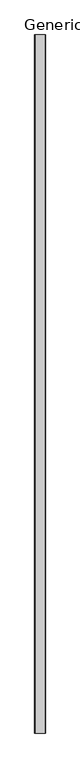
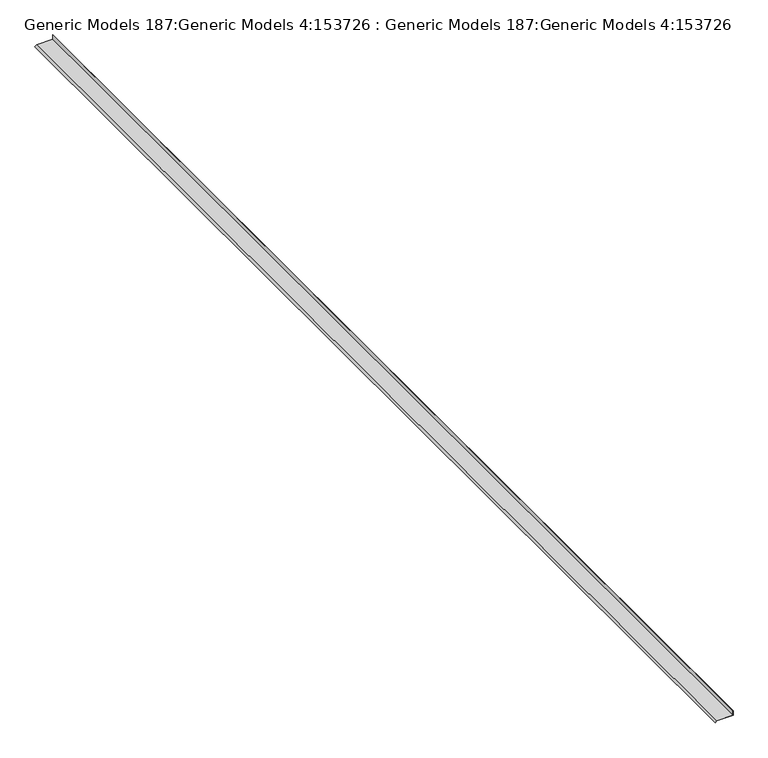
"""IFC4 building model written with IfcOpenShell, lengths in millimetres: proxy geometry, Generic Models 187:Generic Models 4:153726 : Generic Models 187:Generic Models 4:153726."""

from ifc_helpers import new_model, si_unit, frame, origin, place, context, project, spatial, polyline, outline, extrude, source, transform, mapped, element, save


def generic_models_187_generic_models_4_153726_generic_models_bf919b30(model_context):
    return source(origin(), model_context, "Body", "SweptSolid", [
        extrude(outline(polyline([(3472.65625, -5352.4936422), (3472.65625, -5243.5819949), (3505.2, -5243.5819949), (3505.2, -5244.3757449), (3473.45, -5244.3757449), (3473.45, -5352.8224242), (3462.2246798, -5364.0477444), (3461.6634138, -5363.4864784), (3472.65625, -5352.4936422)])), frame((0.0, -273.9974793, 0.0), z_axis=(0.0, 1.0, 0.0), x_axis=(0.0, 0.0, 1.0)), (0.0, 0.0, 1.0), 7886.7),
    ])


if __name__ == "__main__":
    model = new_model("IFC4")
    model_context = context("Model", 3, world=origin())
    ifc_project = project(units=[si_unit("LENGTHUNIT", "METRE", prefix="MILLI")], contexts=[model_context])
    site = spatial("IfcSite", under=ifc_project)
    building = spatial("IfcBuilding", under=site)
    placement = place(None, origin())
    generic_models_187_generic_models_4_153726_generic_models_shape = generic_models_187_generic_models_4_153726_generic_models_bf919b30(model_context)
    element("IfcBuildingElementProxy", 1, Name="Generic Models 187:Generic Models 4:153726 : Generic Models 187:Generic Models 4:153726", ObjectType="Generic Models 187:Generic Models 4:153726 : Generic Models 187:Generic Models 4:153726", at=placement, inside=building, context=model_context, shape_type="MappedRepresentation", body=[
        mapped(generic_models_187_generic_models_4_153726_generic_models_shape, transform((0.0, 0.0, 0.0), x_axis=(1.0, 0.0, 0.0), y_axis=(0.0, 1.0, 0.0), z_axis=(0.0, 0.0, 1.0))),
    ])
    save(model, "model.ifc")

# Revit data of these elements
# Type "Generic Models 187:Generic Models 4:153726 : Generic Models 187:Generic Models 4:153726"
#   NameOverride = "Generic Models 187:Generic Models 4:153726"
#   ObjectTypeOverride = "Generic Models 187:Generic Models 4"
#   Reference = "Generic Models 4"
#   Category = "Generic Models"
#   Tag = "153726"
# Element 1 (IfcBuildingElementProxy, "Generic Models 187:Generic Models 4:153726 : Generic Models 187:Generic Models 4:153726")
#   Materials on its faces: "_12 GAUGE S.S. FLASHING WITH END DAMS 16315"
# Materials
#   "_12 GAUGE S.S. FLASHING WITH END DAMS 16315": class "Unassigned", colour RGB 67 154 161, transparency 0
